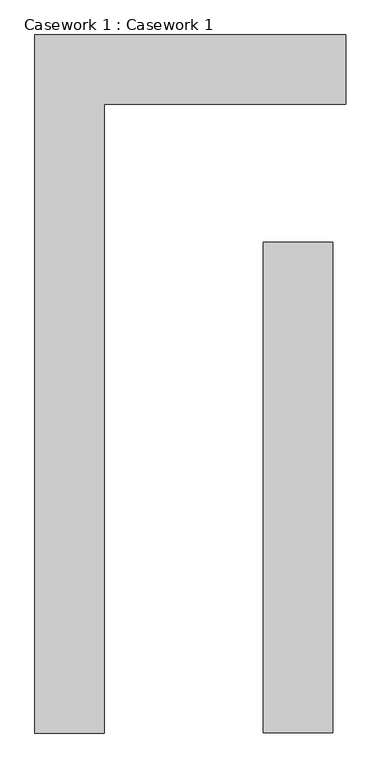
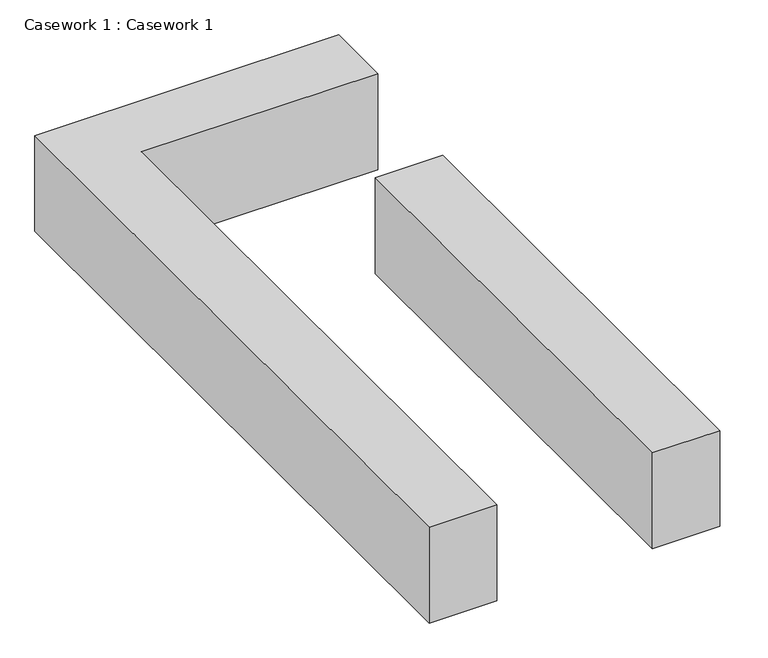
"""IFC4 building model written with IfcOpenShell, lengths in millimetres: furniture geometry, Casework 1 : Casework 1."""

import ifcopenshell
import ifcopenshell.guid

model = None  # the IFC model being written
_history = None  # IfcOwnerHistory: only IFC2X3 demands one
_inside = {}  # id of a spatial element -> (the spatial element, [elements in it])
_under = {}  # id of a project, library or spatial element -> (it, [spatial elements below it])
_declared = {}  # id of a project -> (the project, [libraries it declares])
_typed = {}  # id of a type object -> (the type object, [elements of that type])
_made_of = {}  # id of a material, layer set ... -> (it, [elements and type objects made of it])


def new_model(schema):
    """Start an empty IFC model of exactly this schema.

    Asked for "IFC4X3", IfcOpenShell would pick the latest addendum, in which some entities
    have other attributes; the version numbers below select the first issue.
    IFC2X3 requires an IfcOwnerHistory on every rooted entity: one is made here for all.
    """
    global model, _history
    if schema == "IFC4X3":
        model = ifcopenshell.file(schema_version=(4, 3, 0, 0))
    else:
        model = ifcopenshell.file(schema=schema)
    _inside.clear()
    _under.clear()
    _declared.clear()
    _typed.clear()
    _made_of.clear()
    _history = None
    if model.schema == "IFC2X3":
        org = make("IfcOrganization", Name="unknown")
        user = make(
            "IfcPersonAndOrganization",
            ThePerson=make("IfcPerson", FamilyName="unknown"),
            TheOrganization=org,
        )
        app = make(
            "IfcApplication",
            ApplicationDeveloper=org,
            Version="unknown",
            ApplicationFullName="unknown",
            ApplicationIdentifier="unknown",
        )
        _history = make(
            "IfcOwnerHistory",
            OwningUser=user,
            OwningApplication=app,
            ChangeAction="ADDED",
            CreationDate=0,
        )
    return model


def make(cls, **values):
    """One entity of the class cls with the attributes given. An attribute that is None is left unset."""
    return model.create_entity(
        cls, **{name: value for name, value in values.items() if value is not None}
    )


def rooted(cls, **values):
    """An entity with a GlobalId (a new one), such as an element, a storey or a relation."""
    return make(cls, GlobalId=ifcopenshell.guid.new(), OwnerHistory=_history, **values)


def si_unit(unit_type, name, prefix=None):
    """IfcSIUnit, for example si_unit("LENGTHUNIT", "METRE", prefix="MILLI")."""
    return make("IfcSIUnit", UnitType=unit_type, Prefix=prefix, Name=name)


def assignment(units):
    """IfcUnitAssignment: the units of a project."""
    return None if units is None else make("IfcUnitAssignment", Units=units)


def point(xyz):
    """IfcCartesianPoint."""
    return None if xyz is None else make("IfcCartesianPoint", Coordinates=xyz)


def direction(xyz):
    """IfcDirection."""
    return None if xyz is None else make("IfcDirection", DirectionRatios=xyz)


def frame(location, z_axis=None, x_axis=None):
    """IfcAxis2Placement3D, a coordinate frame: its origin and axes. An axis left out is left unset."""
    return make(
        "IfcAxis2Placement3D",
        Location=point(location),
        Axis=direction(z_axis),
        RefDirection=direction(x_axis),
    )


def origin():
    """The frame at (0, 0, 0) with its axes left unset."""
    return frame((0.0, 0.0, 0.0))


def origin_with_axes():
    """The frame at (0, 0, 0) with the z axis (0, 0, 1) and the x axis (1, 0, 0) written out."""
    return frame((0.0, 0.0, 0.0), z_axis=(0.0, 0.0, 1.0), x_axis=(1.0, 0.0, 0.0))


def place(relative_to, where):
    """IfcLocalPlacement: puts the frame where relative to a parent placement (None: the world)."""
    return make(
        "IfcLocalPlacement", PlacementRelTo=relative_to, RelativePlacement=where
    )


def context(
    kind, dimensions, precision=None, world=None, true_north=None, identifier=None
):
    """IfcGeometricRepresentationContext, for example the 3D "Model" context."""
    return make(
        "IfcGeometricRepresentationContext",
        ContextIdentifier=identifier,
        ContextType=kind,
        CoordinateSpaceDimension=dimensions,
        Precision=precision,
        WorldCoordinateSystem=world,
        TrueNorth=true_north,
    )


def project(units=None, contexts=None):
    """IfcProject with its units and contexts."""
    return rooted(
        "IfcProject",
        Name="project",
        RepresentationContexts=contexts,
        UnitsInContext=assignment(units),
    )


def spatial(cls, under=None, at=None, **own):
    """A site, building, storey or space (cls), placed at a placement, below another one or the project."""
    s = rooted(cls, ObjectPlacement=at, **own)
    if under is not None:
        _under.setdefault(under.id(), (under, []))[1].append(s)
    return s


def polyline(points):
    """IfcPolyline through the points."""
    return make("IfcPolyline", Points=[point(p) for p in points])


def outline(outer, holes=None, kind="AREA"):
    """IfcArbitraryClosedProfileDef: a profile drawn as a closed curve; with holes, ...WithVoids."""
    if holes is None:
        return make("IfcArbitraryClosedProfileDef", ProfileType=kind, OuterCurve=outer)
    return make(
        "IfcArbitraryProfileDefWithVoids",
        ProfileType=kind,
        OuterCurve=outer,
        InnerCurves=holes,
    )


def extrude(swept, where, along, depth):
    """IfcExtrudedAreaSolid: the profile swept, set in the frame where, extruded along a direction by depth."""
    return make(
        "IfcExtrudedAreaSolid",
        SweptArea=swept,
        Position=where,
        ExtrudedDirection=direction(along),
        Depth=depth,
    )


def shape(context_of_items, identifier, shape_type, items):
    """IfcShapeRepresentation: the items that make up one representation, for example the "Body"."""
    return make(
        "IfcShapeRepresentation",
        ContextOfItems=context_of_items,
        RepresentationIdentifier=identifier,
        RepresentationType=shape_type,
        Items=items,
    )


def source(mapping_origin, context_of_items, identifier, shape_type, items):
    """IfcRepresentationMap: a shape defined once, which mapped items show again and again."""
    return make(
        "IfcRepresentationMap",
        MappingOrigin=mapping_origin,
        MappedRepresentation=shape(context_of_items, identifier, shape_type, items),
    )


def transform(
    local_origin,
    x_axis=None,
    y_axis=None,
    z_axis=None,
    scale=None,
    scale2=None,
    scale3=None,
    uniform=True,
):
    """IfcCartesianTransformationOperator3D, or its non-uniform kind. x_axis, y_axis, z_axis: its Axis1, 2, 3."""
    if uniform:
        return make(
            "IfcCartesianTransformationOperator3D",
            Axis1=direction(x_axis),
            Axis2=direction(y_axis),
            LocalOrigin=point(local_origin),
            Scale=scale,
            Axis3=direction(z_axis),
        )
    return make(
        "IfcCartesianTransformationOperator3DnonUniform",
        Axis1=direction(x_axis),
        Axis2=direction(y_axis),
        LocalOrigin=point(local_origin),
        Scale=scale,
        Axis3=direction(z_axis),
        Scale2=scale2,
        Scale3=scale3,
    )


def mapped(mapping_source, mapping_target):
    """IfcMappedItem: shows the shape of a source again, moved by a transform."""
    return make(
        "IfcMappedItem", MappingSource=mapping_source, MappingTarget=mapping_target
    )


def made_of(thing, what):
    """Note that an element or type object is made of a material, layer set ...; save() writes the relation."""
    if what is not None:
        _made_of.setdefault(what.id(), (what, []))[1].append(thing)
    return thing


def element(
    cls,
    number,
    at=None,
    inside=None,
    cuts=None,
    type_object=None,
    material=None,
    context=None,
    identifier="Body",
    shape_type=None,
    held_by="IfcProductDefinitionShape",
    body=None,
    shapes=None,
    **own,
):
    """One element of the class cls, such as IfcWall. Its Tag is "e" and its number.

    at: its placement. inside: the storey or other place that contains it. cuts: it is an
    opening in that element (IfcRelVoidsElement). A single representation is given by context,
    identifier, shape_type and body (its items); several are given by shapes. held_by: the class
    of the entity that holds the representations. save() writes the other relations.
    """
    e = rooted(cls, Tag="e%d" % number, ObjectPlacement=at, **own)
    if body is not None:
        shapes = [shape(context, identifier, shape_type, body)]
    if shapes is not None:
        e.Representation = make(held_by, Representations=shapes)
    if inside is not None:
        _inside.setdefault(inside.id(), (inside, []))[1].append(e)
    if cuts is not None:
        rooted(
            "IfcRelVoidsElement", RelatingBuildingElement=cuts, RelatedOpeningElement=e
        )
    if type_object is not None:
        _typed.setdefault(type_object.id(), (type_object, []))[1].append(e)
    return made_of(e, material)


def aggregate(whole, parts):
    """IfcRelAggregates: a whole, such as a stair, and the parts it consists of."""
    return rooted("IfcRelAggregates", RelatingObject=whole, RelatedObjects=parts)


def save(model, path):
    """Write the relations noted so far, then the file.

    IfcRelAggregates (storeys below a building ...), IfcRelContainedInSpatialStructure (elements
    in a storey), IfcRelDefinesByType, IfcRelAssociatesMaterial and IfcRelDeclares: one each for
    every whole, place, type object, material and project.
    """
    for whole, parts in _under.values():
        aggregate(whole, parts)
    for where, things in _inside.values():
        rooted(
            "IfcRelContainedInSpatialStructure",
            RelatedElements=things,
            RelatingStructure=where,
        )
    for kind, things in _typed.values():
        rooted("IfcRelDefinesByType", RelatedObjects=things, RelatingType=kind)
    for what, things in _made_of.values():
        rooted("IfcRelAssociatesMaterial", RelatedObjects=things, RelatingMaterial=what)
    for by, libraries in _declared.values():
        rooted("IfcRelDeclares", RelatingContext=by, RelatedDefinitions=libraries)
    model.write(path)


def casework_1_casework_1_d615d7ec(model_context):
    return source(origin(), model_context, "Body", "SweptSolid", [
        extrude(outline(polyline([(653847.1867239, -574091.7445091), (653847.1867239, -567932.6413841), (656590.3867239, -567932.6413841), (656590.3867239, -568542.2413841), (654456.7867239, -568542.2413841), (654456.7867239, -574091.7445091), (653847.1867239, -574091.7445091)])), origin_with_axes(), (0.0, 0.0, 1.0), 914.4),
        extrude(outline(polyline([(655863.3117239, -574088.9663841), (655863.3117239, -569761.4413841), (656472.9117239, -569761.4413841), (656472.9117239, -574088.9663841), (655863.3117239, -574088.9663841)])), origin_with_axes(), (0.0, 0.0, 1.0), 914.4),
    ])


if __name__ == "__main__":
    model = new_model("IFC4")
    model_context = context("Model", 3, world=origin())
    ifc_project = project(units=[si_unit("LENGTHUNIT", "METRE", prefix="MILLI")], contexts=[model_context])
    site = spatial("IfcSite", under=ifc_project)
    building = spatial("IfcBuilding", under=site)
    placement = place(None, origin())
    casework_1_casework_1_shape = casework_1_casework_1_d615d7ec(model_context)
    element("IfcFurniture", 1, ObjectType="Casework 1 : Casework 1", at=placement, inside=building, context=model_context, shape_type="MappedRepresentation", body=[
        mapped(casework_1_casework_1_shape, transform((0.0, 0.0, 0.0), x_axis=(1.0, 0.0, 0.0), y_axis=(0.0, 1.0, 0.0), z_axis=(0.0, 0.0, 1.0))),
    ])
    save(model, "model.ifc")

# Revit data of these elements
# Element 1 (IfcFurniture, "Casework 1 : Casework 1")
#   Materials on its faces: "INTERIOR PLYWOOD - SEE DETAILS"
# Materials
#   "INTERIOR PLYWOOD - SEE DETAILS": class "Wood", colour RGB 212 179 113, transparency 0, Description = "Plywood, sheathing grade", Cost = 0
